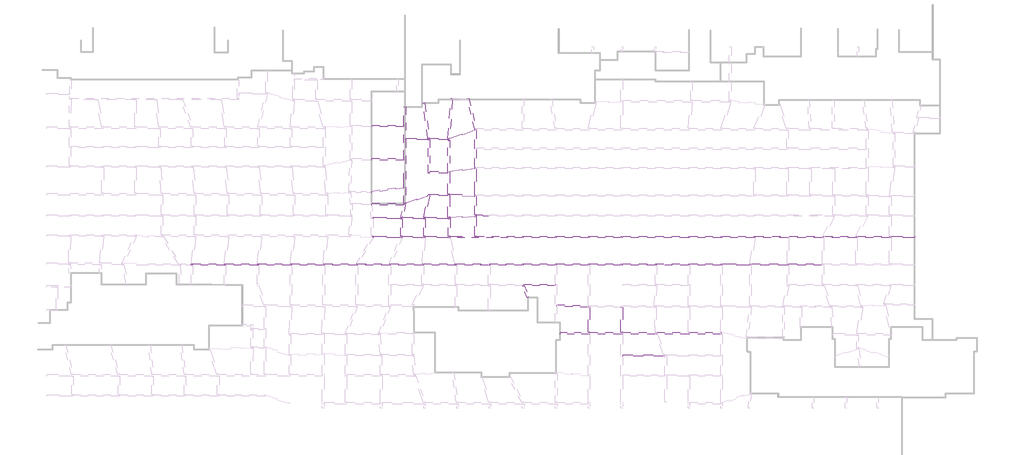
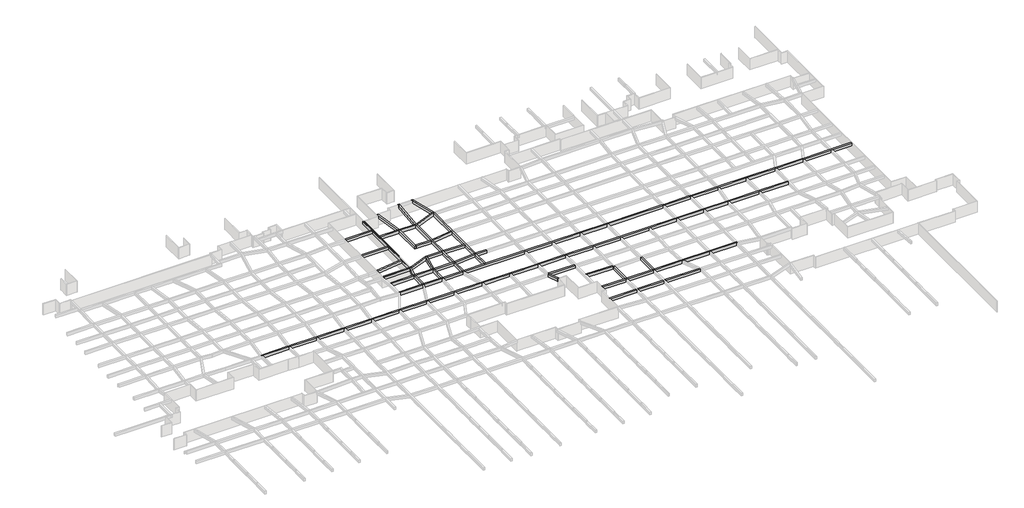
# One storey, part 38 of 45: 38 beams.
"""IFC4 building model written with IfcOpenShell, lengths in millimetres."""

from ifc_helpers import new_model, si_unit, frame, origin, place, context, project, spatial, polyline, outline, extrude, faceted_brep, element, save

model = new_model("IFC4")

# Units and contexts
model_context = context("Model", 3, world=origin())
ifc_project = project(units=[si_unit("LENGTHUNIT", "METRE", prefix="MILLI")], contexts=[model_context])

# Site, building, storey
site = spatial("IfcSite", under=ifc_project)
building = spatial("IfcBuilding", under=site)
storey = spatial("IfcBuildingStorey", under=building, Name="户型图", Elevation=0.0)

# Beams
placement = place(None, origin())
element("IfcBeam", 1, ObjectType="混凝土 - 矩形梁 : KL_beam", at=placement, inside=storey, context=model_context, shape_type="Brep", body=[
    faceted_brep([(-107399.1449794, 152479.7935386, 3300.0), (-107399.1449794, 152079.7935386, 3300.0), (-107019.2456688, 152079.7935386, 3300.0), (-99643.5692432, 152079.7935386, 3300.0), (-99243.5692432, 152079.7935386, 3300.0), (-91843.5387872, 152079.7935386, 3300.0), (-91443.5387872, 152079.7935386, 3300.0), (-84024.3638582, 152079.7935386, 3300.0), (-83624.3638582, 152079.7935386, 3300.0), (-76287.7540188, 152079.7935386, 3300.0), (-75887.7540188, 152079.7935386, 3300.0), (-68487.7540188, 152079.7935386, 3300.0), (-68087.7540188, 152079.7935386, 3300.0), (-60687.7540188, 152079.7935386, 3300.0), (-60287.7540188, 152079.7935386, 3300.0), (-52887.7424309, 152079.7935386, 3300.0), (-52487.7424309, 152079.7935386, 3300.0), (-45087.7540188, 152079.7935386, 3300.0), (-44687.7540188, 152079.7935386, 3300.0), (-37220.6748317, 152079.7935386, 3300.0), (-36820.6748317, 152079.7935386, 3300.0), (-29220.6748317, 152079.7935386, 3300.0), (-28820.6748317, 152079.7935386, 3300.0), (-21420.6748317, 152079.7935386, 3300.0), (-21020.6748317, 152079.7935386, 3300.0), (-13620.6748317, 152079.7935386, 3300.0), (-13220.6748317, 152079.7935386, 3300.0), (-5904.3123934, 152079.7935386, 3300.0), (-5504.3123934, 152079.7935386, 3300.0), (2173.6750398, 152079.7935386, 3300.0), (2573.6750398, 152079.7935386, 3300.0), (9973.3027926, 152079.7935386, 3300.0), (10373.3027926, 152079.7935386, 3300.0), (17658.170888, 152079.7935386, 3300.0), (18058.170888, 152079.7935386, 3300.0), (24544.7928364, 152079.7935386, 3300.0), (24944.7928364, 152079.7935386, 3300.0), (33358.170888, 152079.7935386, 3300.0), (33758.170888, 152079.7935386, 3300.0), (41658.170888, 152079.7935386, 3300.0), (41658.170888, 152479.7935386, 3300.0), (33758.170888, 152479.7935386, 3300.0), (33358.170888, 152479.7935386, 3300.0), (24974.8665178, 152479.7935386, 3300.0), (24570.9354888, 152479.7935386, 3300.0), (18058.170888, 152479.7935386, 3300.0), (17658.170888, 152479.7935386, 3300.0), (10373.3027926, 152479.7935386, 3300.0), (9973.3027926, 152479.7935386, 3300.0), (-5504.3123934, 152479.7935386, 3300.0), (-5904.3123934, 152479.7935386, 3300.0), (-13220.6748317, 152479.7935386, 3300.0), (-13620.6748317, 152479.7935386, 3300.0), (-21020.6748317, 152479.7935386, 3300.0), (-21420.6748317, 152479.7935386, 3300.0), (-28820.6748317, 152479.7935386, 3300.0), (-29220.6748317, 152479.7935386, 3300.0), (-44731.4968935, 152479.7935386, 3300.0), (-45143.7423452, 152479.7935386, 3300.0), (-52476.9979937, 152479.7935386, 3300.0), (-52877.5469321, 152479.7935386, 3300.0), (-60185.5869801, 152479.7935386, 3300.0), (-60620.131131, 152479.7935386, 3300.0), (-67941.3438573, 152479.7935386, 3300.0), (-68403.2240726, 152479.7935386, 3300.0), (-75865.4450548, 152479.7935386, 3300.0), (-76267.6837854, 152479.7935386, 3300.0), (-83602.0244383, 152479.7935386, 3300.0), (-84004.2631688, 152479.7935386, 3300.0), (-91421.2298232, 152479.7935386, 3300.0), (-91823.4685538, 152479.7935386, 3300.0), (-99221.2298232, 152479.7935386, 3300.0), (-99623.4685538, 152479.7935386, 3300.0), (-106996.9062488, 152479.7935386, 3300.0), (-107399.1449794, 152079.7935386, 2500.0), (-107019.2456688, 152079.7935386, 2500.0), (-99643.5692432, 152079.7935386, 2500.0), (-99243.5692432, 152079.7935386, 2500.0), (-91843.5387872, 152079.7935386, 2500.0), (-91443.5387872, 152079.7935386, 2500.0), (-84024.3638582, 152079.7935386, 2500.0), (-83624.3638582, 152079.7935386, 2500.0), (-76287.7540188, 152079.7935386, 2500.0), (-75887.7540188, 152079.7935386, 2500.0), (-68487.7540188, 152079.7935386, 2500.0), (-68087.7540188, 152079.7935386, 2500.0), (-60687.7540188, 152079.7935386, 2500.0), (-60287.7540188, 152079.7935386, 2500.0), (-52887.7424309, 152079.7935386, 2500.0), (-52487.7424309, 152079.7935386, 2500.0), (-45087.7540188, 152079.7935386, 2500.0), (-44687.7540188, 152079.7935386, 2500.0), (-37220.6748317, 152079.7935386, 2500.0), (-36820.6748317, 152079.7935386, 2500.0), (-29220.6748317, 152079.7935386, 2500.0), (-28820.6748317, 152079.7935386, 2500.0), (-21420.6748317, 152079.7935386, 2500.0), (-21020.6748317, 152079.7935386, 2500.0), (-13620.6748317, 152079.7935386, 2500.0), (-13220.6748317, 152079.7935386, 2500.0), (-5904.3123934, 152079.7935386, 2500.0), (-5504.3123934, 152079.7935386, 2500.0), (2173.6750398, 152079.7935386, 2500.0), (2573.6750398, 152079.7935386, 2500.0), (9973.3027926, 152079.7935386, 2500.0), (10373.3027926, 152079.7935386, 2500.0), (17658.170888, 152079.7935386, 2500.0), (18058.170888, 152079.7935386, 2500.0), (24544.7928364, 152079.7935386, 2500.0), (24944.7928364, 152079.7935386, 2500.0), (33358.170888, 152079.7935386, 2500.0), (33758.170888, 152079.7935386, 2500.0), (41658.170888, 152079.7935386, 2500.0), (-107399.1449794, 152479.7935386, 2500.0), (-106996.9062488, 152479.7935386, 2500.0), (-99623.4685538, 152479.7935386, 2500.0), (-99221.2298232, 152479.7935386, 2500.0), (-91823.4685538, 152479.7935386, 2500.0), (-91421.2298232, 152479.7935386, 2500.0), (-84004.2631688, 152479.7935386, 2500.0), (-83602.0244383, 152479.7935386, 2500.0), (-76267.6837854, 152479.7935386, 2500.0), (-75865.4450548, 152479.7935386, 2500.0), (-68403.2240726, 152479.7935386, 2500.0), (-67941.3438573, 152479.7935386, 2500.0), (-60620.131131, 152479.7935386, 2500.0), (-60185.5869801, 152479.7935386, 2500.0), (-52877.5469321, 152479.7935386, 2500.0), (-52476.9979937, 152479.7935386, 2500.0), (-45143.7423452, 152479.7935386, 2500.0), (-44731.4968935, 152479.7935386, 2500.0), (-29220.6748317, 152479.7935386, 2500.0), (-28820.6748317, 152479.7935386, 2500.0), (-21420.6748317, 152479.7935386, 2500.0), (-21020.6748317, 152479.7935386, 2500.0), (-13620.6748317, 152479.7935386, 2500.0), (-13220.6748317, 152479.7935386, 2500.0), (-5904.3123934, 152479.7935386, 2500.0), (-5504.3123934, 152479.7935386, 2500.0), (9973.3027926, 152479.7935386, 2500.0), (10373.3027926, 152479.7935386, 2500.0), (17658.170888, 152479.7935386, 2500.0), (18058.170888, 152479.7935386, 2500.0), (24570.9354888, 152479.7935386, 2500.0), (24974.8665178, 152479.7935386, 2500.0), (33358.170888, 152479.7935386, 2500.0), (33758.170888, 152479.7935386, 2500.0), (41658.170888, 152479.7935386, 2500.0)], [[[0, 1, 2, 3, 4, 5, 6, 7, 8, 9, 10, 11, 12, 13, 14, 15, 16, 17, 18, 19, 20, 21, 22, 23, 24, 25, 26, 27, 28, 29, 30, 31, 32, 33, 34, 35, 36, 37, 38, 39, 40, 41, 42, 43, 44, 45, 46, 47, 48, 49, 50, 51, 52, 53, 54, 55, 56, 57, 58, 59, 60, 61, 62, 63, 64, 65, 66, 67, 68, 69, 70, 71, 72, 73]], [[1, 74, 75, 76, 77, 78, 79, 80, 81, 82, 83, 84, 85, 86, 87, 88, 89, 90, 91, 92, 93, 94, 95, 96, 97, 98, 99, 100, 101, 102, 103, 104, 105, 106, 107, 108, 109, 110, 111, 112, 39, 38, 37, 36, 35, 34, 33, 32, 31, 30, 29, 28, 27, 26, 25, 24, 23, 22, 21, 20, 19, 18, 17, 16, 15, 14, 13, 12, 11, 10, 9, 8, 7, 6, 5, 4, 3, 2]], [[74, 113, 114, 115, 116, 117, 118, 119, 120, 121, 122, 123, 124, 125, 126, 127, 128, 129, 130, 131, 132, 133, 134, 135, 136, 137, 138, 139, 140, 141, 142, 143, 144, 145, 146, 147, 112, 111, 110, 109, 108, 107, 106, 105, 104, 103, 102, 101, 100, 99, 98, 97, 96, 95, 94, 93, 92, 91, 90, 89, 88, 87, 86, 85, 84, 83, 82, 81, 80, 79, 78, 77, 76, 75]], [[113, 0, 73, 72, 71, 70, 69, 68, 67, 66, 65, 64, 63, 62, 61, 60, 59, 58, 57, 56, 55, 54, 53, 52, 51, 50, 49, 48, 47, 46, 45, 44, 43, 42, 41, 40, 147, 146, 145, 144, 143, 142, 141, 140, 139, 138, 137, 136, 135, 134, 133, 132, 131, 130, 129, 128, 127, 126, 125, 124, 123, 122, 121, 120, 119, 118, 117, 116, 115, 114]], [[0, 113, 74, 1]], [[40, 39, 112, 147]]]),
])
element("IfcBeam", 2, ObjectType="混凝土 - 矩形梁 : KL_beam", at=placement, inside=storey, context=model_context, shape_type="Brep", body=[
    faceted_brep([(63459.1822514, 158978.3181414, 3300.0), (63459.1822514, 158578.3181414, 3300.0), (63459.1822514, 158578.3181414, 2500.0), (63459.1822514, 158978.3181414, 2500.0), (57931.1254195, 158978.3181414, 3300.0), (57531.1254195, 158978.3181414, 3300.0), (50062.8813826, 158978.3181414, 3300.0), (49613.9508875, 158978.3181414, 3300.0), (42278.2377938, 158978.3181414, 3300.0), (41833.1970176, 158978.3181414, 3300.0), (25858.170888, 158978.3181414, 3300.0), (25458.170888, 158978.3181414, 3300.0), (18058.170888, 158978.3181414, 3300.0), (17658.170888, 158978.3181414, 3300.0), (10373.3027926, 158978.3181414, 3300.0), (9973.3027926, 158978.3181414, 3300.0), (-5504.3123934, 158978.3181414, 3300.0), (-5904.3123934, 158978.3181414, 3300.0), (-13220.6748317, 158978.3181414, 3300.0), (-13620.6748317, 158978.3181414, 3300.0), (-21020.6748317, 158978.3181414, 3300.0), (-21420.6748317, 158978.3181414, 3300.0), (-28820.6748317, 158978.3181414, 3300.0), (-29220.6748317, 158978.3181414, 3300.0), (-40021.1080966, 158978.3181414, 3300.0), (-40421.1080966, 158978.3181414, 3300.0), (-46244.2344007, 158978.3181414, 3300.0), (-46644.2344007, 158978.3181414, 3300.0), (-52129.2939824, 158978.3181414, 3300.0), (-52529.2939824, 158978.3181414, 3300.0), (-57529.2939824, 158978.3181414, 3300.0), (-57929.2939824, 158978.3181414, 3300.0), (-64444.2344007, 158978.3181414, 3300.0), (-64637.1523876, 158978.3181414, 3300.0), (-64301.3522933, 158784.4438666, 3300.0), (-64420.3590362, 158578.3181414, 3300.0), (-58031.4610211, 158578.3181414, 3300.0), (-57596.9168701, 158578.3181414, 3300.0), (-52557.9368008, 158578.3181414, 3300.0), (-52157.3878624, 158578.3181414, 3300.0), (-46664.2753047, 158578.3181414, 3300.0), (-46252.029853, 158578.3181414, 3300.0), (-46244.2344007, 158578.3181414, 3300.0), (-29220.6748317, 158578.3181414, 3300.0), (-28820.6748317, 158578.3181414, 3300.0), (-21420.6748317, 158578.3181414, 3300.0), (-21020.6748317, 158578.3181414, 3300.0), (-13620.6748317, 158578.3181414, 3300.0), (-13220.6748317, 158578.3181414, 3300.0), (-5904.3123934, 158578.3181414, 3300.0), (-5504.3123934, 158578.3181414, 3300.0), (9973.3027926, 158578.3181414, 3300.0), (10373.3027926, 158578.3181414, 3300.0), (17658.170888, 158578.3181414, 3300.0), (18058.170888, 158578.3181414, 3300.0), (25428.027227, 158578.3181414, 3300.0), (25831.958256, 158578.3181414, 3300.0), (33358.170888, 158578.3181414, 3300.0), (33758.170888, 158578.3181414, 3300.0), (41658.170888, 158578.3181414, 3300.0), (42058.170888, 158578.3181414, 3300.0), (49536.7318858, 158578.3181414, 3300.0), (49936.7318858, 158578.3181414, 3300.0), (57531.1254195, 158578.3181414, 3300.0), (57931.1254195, 158578.3181414, 3300.0), (-64420.3590362, 158578.3181414, 2500.0), (-58031.4610211, 158578.3181414, 2500.0), (-57596.9168701, 158578.3181414, 2500.0), (-52557.9368008, 158578.3181414, 2500.0), (-52157.3878624, 158578.3181414, 2500.0), (-46664.2753047, 158578.3181414, 2500.0), (-46252.029853, 158578.3181414, 2500.0), (-46244.2344007, 158578.3181414, 2500.0), (-29220.6748317, 158578.3181414, 2500.0), (-28820.6748317, 158578.3181414, 2500.0), (-21420.6748317, 158578.3181414, 2500.0), (-21020.6748317, 158578.3181414, 2500.0), (-13620.6748317, 158578.3181414, 2500.0), (-13220.6748317, 158578.3181414, 2500.0), (-5904.3123934, 158578.3181414, 2500.0), (-5504.3123934, 158578.3181414, 2500.0), (9973.3027926, 158578.3181414, 2500.0), (10373.3027926, 158578.3181414, 2500.0), (17658.170888, 158578.3181414, 2500.0), (18058.170888, 158578.3181414, 2500.0), (25428.027227, 158578.3181414, 2500.0), (25831.958256, 158578.3181414, 2500.0), (33358.170888, 158578.3181414, 2500.0), (33758.170888, 158578.3181414, 2500.0), (41658.170888, 158578.3181414, 2500.0), (42058.170888, 158578.3181414, 2500.0), (49536.7318858, 158578.3181414, 2500.0), (49936.7318858, 158578.3181414, 2500.0), (57531.1254195, 158578.3181414, 2500.0), (57931.1254195, 158578.3181414, 2500.0), (-64301.3522933, 158784.4438666, 2500.0), (-64637.1523876, 158978.3181414, 2500.0), (-64444.2344007, 158978.3181414, 2500.0), (-57929.2939824, 158978.3181414, 2500.0), (-57529.2939824, 158978.3181414, 2500.0), (-52529.2939824, 158978.3181414, 2500.0), (-52129.2939824, 158978.3181414, 2500.0), (-46644.2344007, 158978.3181414, 2500.0), (-46244.2344007, 158978.3181414, 2500.0), (-40421.1080966, 158978.3181414, 2500.0), (-40021.1080966, 158978.3181414, 2500.0), (-29220.6748317, 158978.3181414, 2500.0), (-28820.6748317, 158978.3181414, 2500.0), (-21420.6748317, 158978.3181414, 2500.0), (-21020.6748317, 158978.3181414, 2500.0), (-13620.6748317, 158978.3181414, 2500.0), (-13220.6748317, 158978.3181414, 2500.0), (-5904.3123934, 158978.3181414, 2500.0), (-5504.3123934, 158978.3181414, 2500.0), (9973.3027926, 158978.3181414, 2500.0), (10373.3027926, 158978.3181414, 2500.0), (17658.170888, 158978.3181414, 2500.0), (18058.170888, 158978.3181414, 2500.0), (25458.170888, 158978.3181414, 2500.0), (25858.170888, 158978.3181414, 2500.0), (41833.1970176, 158978.3181414, 2500.0), (42278.2377938, 158978.3181414, 2500.0), (49613.9508875, 158978.3181414, 2500.0), (50062.8813826, 158978.3181414, 2500.0), (57531.1254195, 158978.3181414, 2500.0), (57931.1254195, 158978.3181414, 2500.0)], [[[0, 1, 2, 3]], [[1, 0, 4, 5, 6, 7, 8, 9, 10, 11, 12, 13, 14, 15, 16, 17, 18, 19, 20, 21, 22, 23, 24, 25, 26, 27, 28, 29, 30, 31, 32, 33, 34, 35, 36, 37, 38, 39, 40, 41, 42, 43, 44, 45, 46, 47, 48, 49, 50, 51, 52, 53, 54, 55, 56, 57, 58, 59, 60, 61, 62, 63, 64]], [[2, 1, 64, 63, 62, 61, 60, 59, 58, 57, 56, 55, 54, 53, 52, 51, 50, 49, 48, 47, 46, 45, 44, 43, 42, 41, 40, 39, 38, 37, 36, 35, 65, 66, 67, 68, 69, 70, 71, 72, 73, 74, 75, 76, 77, 78, 79, 80, 81, 82, 83, 84, 85, 86, 87, 88, 89, 90, 91, 92, 93, 94]], [[3, 2, 94, 93, 92, 91, 90, 89, 88, 87, 86, 85, 84, 83, 82, 81, 80, 79, 78, 77, 76, 75, 74, 73, 72, 71, 70, 69, 68, 67, 66, 65, 95, 96, 97, 98, 99, 100, 101, 102, 103, 104, 105, 106, 107, 108, 109, 110, 111, 112, 113, 114, 115, 116, 117, 118, 119, 120, 121, 122, 123, 124, 125]], [[0, 3, 125, 124, 123, 122, 121, 120, 119, 118, 117, 116, 115, 114, 113, 112, 111, 110, 109, 108, 107, 106, 105, 104, 103, 102, 101, 100, 99, 98, 97, 96, 33, 32, 31, 30, 29, 28, 27, 26, 25, 24, 23, 22, 21, 20, 19, 18, 17, 16, 15, 14, 13, 12, 11, 10, 9, 8, 7, 6, 5, 4]], [[34, 95, 65, 35]], [[95, 34, 33, 96]]]),
])
element("IfcBeam", 3, ObjectType="混凝土 - 矩形梁 : KL_beam", at=placement, inside=storey, context=model_context, shape_type="Brep", body=[
    faceted_brep([(-64444.2344007, 163210.8437885, 3300.0), (-64444.2344007, 163000.3622326, 3300.0), (-57929.2939824, 163000.3622326, 3300.0), (-57529.2939824, 163000.3622326, 3300.0), (-52529.2939824, 163000.3622326, 3300.0), (-52129.2939824, 163000.3622326, 3300.0), (-46644.2344007, 163000.3622326, 3300.0), (-46244.2344007, 163000.3622326, 3300.0), (-46244.2344007, 163018.5507812, 3300.0), (-46244.2344007, 163400.3622326, 3300.0), (-46344.2344007, 163400.3622326, 3300.0), (-46744.2344007, 163400.3622326, 3300.0), (-52086.6745815, 163400.3622326, 3300.0), (-52494.1612595, 163400.3622326, 3300.0), (-57477.854433, 163400.3622326, 3300.0), (-57888.3760761, 163400.3622326, 3300.0), (-64464.1535918, 163400.3622326, 3300.0), (-64444.2344007, 163000.3622326, 2500.0), (-57929.2939824, 163000.3622326, 2500.0), (-57529.2939824, 163000.3622326, 2500.0), (-52529.2939824, 163000.3622326, 2500.0), (-52129.2939824, 163000.3622326, 2500.0), (-46644.2344007, 163000.3622326, 2500.0), (-46244.2344007, 163000.3622326, 2500.0), (-64444.2344007, 163210.8437885, 2500.0), (-64464.1535918, 163400.3622326, 2500.0), (-57888.3760761, 163400.3622326, 2500.0), (-57477.854433, 163400.3622326, 2500.0), (-52494.1612595, 163400.3622326, 2500.0), (-52086.6745815, 163400.3622326, 2500.0), (-46744.2344007, 163400.3622326, 2500.0), (-46344.2344007, 163400.3622326, 2500.0), (-46244.2344007, 163400.3622326, 2500.0), (-46244.2344007, 163018.5507812, 2500.0)], [[[0, 1, 2, 3, 4, 5, 6, 7, 8, 9, 10, 11, 12, 13, 14, 15, 16]], [[1, 17, 18, 19, 20, 21, 22, 23, 7, 6, 5, 4, 3, 2]], [[17, 24, 25, 26, 27, 28, 29, 30, 31, 32, 33, 23, 22, 21, 20, 19, 18]], [[9, 32, 31, 30, 29, 28, 27, 26, 25, 16, 15, 14, 13, 12, 11, 10]], [[1, 0, 24, 17]], [[0, 16, 25, 24]], [[9, 8, 7, 23, 33, 32]]]),
])
element("IfcBeam", 4, ObjectType="混凝土 - 矩形梁 : KL_beam", at=placement, inside=storey, context=model_context, shape_type="SweptSolid", body=[
    extrude(outline(polyline([(-57529.2939824, 158978.3181414), (-57929.2939824, 158978.3181414), (-57929.2939824, 163000.3622326), (-57529.2939824, 163000.3622326), (-57529.2939824, 158978.3181414)])), frame((0.0, 0.0, 2500.0), z_axis=(0.0, 0.0, 1.0), x_axis=(1.0, 0.0, 0.0)), (0.0, 0.0, 1.0), 800.0),
])
element("IfcBeam", 5, ObjectType="混凝土 - 矩形梁 : KL_beam", at=placement, inside=storey, context=model_context, shape_type="SweptSolid", body=[
    extrude(outline(polyline([(-52129.2939824, 158978.3181414), (-52529.2939824, 158978.3181414), (-52529.2939824, 163000.3622326), (-52129.2939824, 163000.3622326), (-52129.2939824, 158978.3181414)])), frame((0.0, 0.0, 2500.0), z_axis=(0.0, 0.0, 1.0), x_axis=(1.0, 0.0, 0.0)), (0.0, 0.0, 1.0), 800.0),
])
element("IfcBeam", 6, ObjectType="混凝土 - 矩形梁 : KL_beam", at=placement, inside=storey, context=model_context, shape_type="SweptSolid", body=[
    extrude(outline(polyline([(-46644.2344007, 163000.3622326), (-46244.2344007, 163000.3622326), (-46244.2344007, 158978.3181414), (-46644.2344007, 158978.3181414), (-46644.2344007, 163000.3622326)])), frame((0.0, 0.0, 2500.0), z_axis=(0.0, 0.0, 1.0), x_axis=(1.0, 0.0, 0.0)), (0.0, 0.0, 1.0), 800.0),
    extrude(outline(polyline([(-46244.2344007, 158547.0522899), (-46252.029853, 158578.3181414), (-46244.2344007, 158578.3181414), (-46244.2344007, 158547.0522899)])), frame((0.0, 0.0, 2500.0), z_axis=(0.0, 0.0, 1.0), x_axis=(1.0, 0.0, 0.0)), (0.0, 0.0, 1.0), 800.0),
])
element("IfcBeam", 7, ObjectType="混凝土 - 矩形梁 : KL_beam", at=placement, inside=storey, context=model_context, shape_type="Brep", body=[
    faceted_brep([(-56685.1558367, 166833.9170778, 3300.0), (-56771.3878839, 166800.8872671, 3300.0), (-57081.0281845, 166682.2844873, 3300.0), (-57135.5017388, 166661.419261, 3300.0), (-57223.0318982, 166282.2844873, 3300.0), (-57888.3760761, 163400.3622326, 3300.0), (-57477.854433, 163400.3622326, 3300.0), (-56793.6389178, 166364.0252292, 3300.0), (-56685.1558367, 166833.9170778, 2500.0), (-57477.854433, 163400.3622326, 2500.0), (-56793.6389178, 166364.0252292, 2500.0), (-57135.5017388, 166661.419261, 2500.0), (-57081.0281845, 166682.2844873, 2500.0), (-56771.3878839, 166800.8872671, 2500.0), (-57888.3760761, 163400.3622326, 2500.0), (-57223.0318982, 166282.2844873, 2500.0)], [[[0, 1, 2, 3, 4, 5, 6, 7]], [[8, 0, 7, 6, 9, 10]], [[11, 12, 13, 8, 10, 9, 14, 15]], [[3, 11, 15, 14, 5, 4]], [[6, 5, 14, 9]], [[3, 2, 1, 0, 8, 13, 12, 11]]]),
])
element("IfcBeam", 8, ObjectType="混凝土 - 矩形梁 : KL_beam", at=placement, inside=storey, context=model_context, shape_type="Brep", body=[
    faceted_brep([(-51297.7565778, 168897.4744599, 3300.0), (-51435.9175617, 168844.5540981, 3300.0), (-51525.8760493, 168381.7577996, 3300.0), (-52494.1612595, 163400.3622326, 3300.0), (-52086.6745815, 163400.3622326, 3300.0), (-51095.8963311, 168497.4744599, 3300.0), (-51018.1442074, 168897.4744599, 3300.0), (-51018.1442074, 168897.4744599, 2500.0), (-52086.6745815, 163400.3622326, 2500.0), (-51095.8963311, 168497.4744599, 2500.0), (-51435.9175617, 168844.5540981, 2500.0), (-51297.7565778, 168897.4744599, 2500.0), (-52494.1612595, 163400.3622326, 2500.0), (-51525.8760493, 168381.7577996, 2500.0)], [[[0, 1, 2, 3, 4, 5, 6]], [[7, 6, 5, 4, 8, 9]], [[10, 11, 7, 9, 8, 12, 13]], [[1, 10, 13, 12, 3, 2]], [[4, 3, 12, 8]], [[0, 11, 10, 1]], [[11, 0, 6, 7]]]),
])
element("IfcBeam", 9, ObjectType="混凝土 - 矩形梁 : KL_beam", at=placement, inside=storey, context=model_context, shape_type="Brep", body=[
    faceted_brep([(-46344.2344007, 168897.4744599, 3300.0), (-46344.4990045, 168897.4744599, 3300.0), (-46541.0079915, 168897.4744599, 3300.0), (-46744.2344007, 168897.4744599, 3300.0), (-46744.2344007, 168497.4744599, 3300.0), (-46744.2344007, 163400.3622326, 3300.0), (-46344.2344007, 163400.3622326, 3300.0), (-46344.2344007, 163410.8212036, 3300.0), (-46344.2344007, 168490.359157, 3300.0), (-46344.2344007, 168890.6029747, 3300.0), (-46344.2344007, 168897.4744599, 2500.0), (-46344.2344007, 163400.3622326, 2500.0), (-46344.2344007, 163410.8212036, 2500.0), (-46344.2344007, 168490.359157, 2500.0), (-46344.2344007, 168890.6029747, 2500.0), (-46744.2344007, 168897.4744599, 2500.0), (-46541.0079915, 168897.4744599, 2500.0), (-46344.4990045, 168897.4744599, 2500.0), (-46744.2344007, 163400.3622326, 2500.0), (-46744.2344007, 168497.4744599, 2500.0)], [[[0, 1, 2, 3, 4, 5, 6, 7, 8, 9]], [[10, 0, 9, 8, 7, 6, 11, 12, 13, 14]], [[15, 16, 17, 10, 14, 13, 12, 11, 18, 19]], [[3, 15, 19, 18, 5, 4]], [[6, 5, 18, 11]], [[3, 2, 1, 0, 10, 17, 16, 15]]]),
])
element("IfcBeam", 10, ObjectType="混凝土 - 矩形梁 : KL_beam", at=placement, inside=storey, context=model_context, shape_type="SweptSolid", body=[
    extrude(outline(polyline([(-56793.6389178, 166364.0252292), (-56685.1558367, 166833.9170778), (-51435.9175617, 168844.5540981), (-51525.8760493, 168381.7577996), (-56793.6389178, 166364.0252292)])), frame((0.0, 0.0, 2500.0), z_axis=(0.0, 0.0, 1.0), x_axis=(1.0, 0.0, 0.0)), (0.0, 0.0, 1.0), 800.0),
])
element("IfcBeam", 11, ObjectType="混凝土 - 矩形梁 : KL_beam", at=placement, inside=storey, context=model_context, shape_type="Brep", body=[
    faceted_brep([(-51018.1442074, 168897.4744599, 3300.0), (-51085.6096548, 168550.3948218, 3300.0), (-51095.8963311, 168497.4744599, 3300.0), (-46744.2344007, 168497.4744599, 3300.0), (-46744.2344007, 168897.4744599, 3300.0), (-46744.4990045, 168897.4744599, 3300.0), (-51095.8963311, 168497.4744599, 2500.0), (-46744.2344007, 168497.4744599, 2500.0), (-51085.6096548, 168550.3948218, 2500.0), (-51018.1442074, 168897.4744599, 2500.0), (-46744.4990045, 168897.4744599, 2500.0), (-46744.2344007, 168897.4744599, 2500.0)], [[[0, 1, 2, 3, 4, 5]], [[2, 6, 7, 3]], [[6, 8, 9, 10, 11, 7]], [[9, 0, 5, 4, 11, 10]], [[6, 2, 1, 0, 9, 8]], [[4, 3, 7, 11]]]),
])
element("IfcBeam", 12, ObjectType="混凝土 - 矩形梁 : KL_beam", at=placement, inside=storey, context=model_context, shape_type="Brep", body=[
    faceted_brep([(-46344.2344007, 168890.6029747, 3300.0), (-46344.2344007, 168490.359157, 3300.0), (-40420.6748317, 168283.5038987, 3300.0), (-40420.6748317, 168683.7477164, 3300.0), (-46344.2344007, 168490.359157, 2500.0), (-40420.6748317, 168283.5038987, 2500.0), (-46344.2344007, 168890.6029747, 2500.0), (-40420.6748317, 168683.7477164, 2500.0)], [[[0, 1, 2, 3]], [[1, 4, 5, 2]], [[4, 6, 7, 5]], [[6, 0, 3, 7]], [[0, 6, 4, 1]], [[3, 2, 5, 7]]]),
    faceted_brep([(-46541.0079915, 168897.4744599, 2500.0), (-46541.0079915, 168897.4744599, 3300.0), (-46744.2344007, 168897.4744599, 3300.0), (-46744.4990045, 168897.4744599, 3300.0), (-46744.4990045, 168897.4744599, 2500.0), (-46744.2344007, 168897.4744599, 2500.0), (-46744.4990045, 168904.5805227, 3300.0), (-46744.4990045, 168904.5805227, 2500.0)], [[[0, 1, 2, 3, 4, 5]], [[6, 7, 4, 3]], [[1, 6, 3, 2]], [[7, 0, 5, 4]], [[1, 0, 7, 6]]]),
])
element("IfcBeam", 13, ObjectType="混凝土 - 矩形梁 : KL_beam", at=placement, inside=storey, context=model_context, shape_type="Brep", body=[
    faceted_brep([(-46244.2344007, 163400.3622326, 3300.0), (-46244.2344007, 163018.5507812, 3300.0), (-40421.1080966, 163574.6111972, 3300.0), (-40021.1080966, 163612.8078899, 3300.0), (-40020.6748317, 163612.8492632, 3300.0), (-40020.6748317, 163994.4687414, 3300.0), (-40020.6748317, 164014.6688587, 3300.0), (-40420.6748317, 163976.4721659, 3300.0), (-46344.2344007, 163410.8212036, 3300.0), (-46344.2344007, 163400.3622326, 3300.0), (-46244.2344007, 163018.5507812, 2500.0), (-40421.1080966, 163574.6111972, 2500.0), (-40021.1080966, 163612.8078899, 2500.0), (-40020.6748317, 163612.8492632, 2500.0), (-46244.2344007, 163400.3622326, 2500.0), (-46344.2344007, 163400.3622326, 2500.0), (-46344.2344007, 163410.8212036, 2500.0), (-40420.6748317, 163976.4721659, 2500.0), (-40020.6748317, 164014.6688587, 2500.0), (-40020.6748317, 163994.4687414, 2500.0)], [[[0, 1, 2, 3, 4, 5, 6, 7, 8, 9]], [[1, 10, 11, 12, 13, 4, 3, 2]], [[10, 14, 15, 16, 17, 18, 19, 13, 12, 11]], [[6, 18, 17, 16, 8, 7]], [[0, 14, 10, 1]], [[14, 0, 9, 15]], [[9, 8, 16, 15]], [[6, 5, 4, 13, 19, 18]]]),
])
element("IfcBeam", 14, ObjectType="混凝土 - 矩形梁 : KL_beam", at=placement, inside=storey, context=model_context, shape_type="Brep", body=[
    faceted_brep([(-40020.6748317, 184219.2176267, 3300.0), (-40420.6748317, 184170.1038023, 3300.0), (-40420.6748317, 183903.6589088, 3300.0), (-40420.6748317, 175230.1542355, 3300.0), (-40420.6748317, 174825.1839588, 3300.0), (-40420.6748317, 168683.7477164, 3300.0), (-40420.6748317, 168283.5038987, 3300.0), (-40420.6748317, 163976.4721659, 3300.0), (-40020.6748317, 164014.6688587, 3300.0), (-40020.6748317, 168316.2365071, 3300.0), (-40020.6748317, 168716.2365071, 3300.0), (-40020.6748317, 174859.2955299, 3300.0), (-40020.6748317, 175259.2955299, 3300.0), (-40020.6748317, 179411.4368869, 3300.0), (-40020.6748317, 179811.4368869, 3300.0), (-40020.6748317, 183994.3140025, 3300.0), (-40020.6748317, 184219.2176267, 2500.0), (-40020.6748317, 164014.6688587, 2500.0), (-40020.6748317, 168316.2365071, 2500.0), (-40020.6748317, 168716.2365071, 2500.0), (-40020.6748317, 174859.2955299, 2500.0), (-40020.6748317, 175259.2955299, 2500.0), (-40020.6748317, 179411.4368869, 2500.0), (-40020.6748317, 179811.4368869, 2500.0), (-40020.6748317, 183994.3140025, 2500.0), (-40420.6748317, 184170.1038023, 2500.0), (-40420.6748317, 163976.4721659, 2500.0), (-40420.6748317, 168283.5038987, 2500.0), (-40420.6748317, 168683.7477164, 2500.0), (-40420.6748317, 174825.1839588, 2500.0), (-40420.6748317, 175230.1542355, 2500.0), (-40420.6748317, 183903.6589088, 2500.0)], [[[0, 1, 2, 3, 4, 5, 6, 7, 8, 9, 10, 11, 12, 13, 14, 15]], [[16, 0, 15, 14, 13, 12, 11, 10, 9, 8, 17, 18, 19, 20, 21, 22, 23, 24]], [[25, 16, 24, 23, 22, 21, 20, 19, 18, 17, 26, 27, 28, 29, 30, 31]], [[1, 25, 31, 30, 29, 28, 27, 26, 7, 6, 5, 4, 3, 2]], [[8, 7, 26, 17]], [[1, 0, 16, 25]]]),
])
element("IfcBeam", 15, ObjectType="混凝土 - 矩形梁 : KL_beam", at=placement, inside=storey, context=model_context, shape_type="Brep", body=[
    faceted_brep([(-40420.6748317, 184170.1038023, 3300.0), (-40020.6748317, 184219.2176267, 3300.0), (-40064.3312613, 184394.3140025, 3300.0), (-41844.548046, 191534.3735401, 3300.0), (-42256.7934978, 191534.3735401, 3300.0), (-42157.0622966, 191134.3735401, 3300.0), (-40457.5408595, 184317.965364, 3300.0), (-40020.6748317, 184219.2176267, 2500.0), (-40064.3312613, 184394.3140025, 2500.0), (-41844.548046, 191534.3735401, 2500.0), (-40420.6748317, 184170.1038023, 2500.0), (-40457.5408595, 184317.965364, 2500.0), (-42157.0622966, 191134.3735401, 2500.0), (-42256.7934978, 191534.3735401, 2500.0)], [[[0, 1, 2, 3, 4, 5, 6]], [[1, 7, 8, 9, 3, 2]], [[7, 10, 11, 12, 13, 9, 8]], [[10, 0, 6, 5, 4, 13, 12, 11]], [[0, 10, 7, 1]], [[4, 3, 9, 13]]]),
])
element("IfcBeam", 16, ObjectType="混凝土 - 矩形梁 : KL_beam", at=placement, inside=storey, context=model_context, shape_type="Brep", body=[
    faceted_brep([(-46616.2994071, 181525.3814597, 3300.0), (-46344.4990045, 181629.715859, 3300.0), (-40420.6748317, 183903.6589088, 3300.0), (-40420.6748317, 184170.1038023, 3300.0), (-40457.5408595, 184317.965364, 3300.0), (-46347.6097756, 182056.9797433, 3300.0), (-46759.6465869, 181898.8136303, 3300.0), (-46667.7042024, 181659.2955299, 3300.0), (-46759.6465869, 181898.8136303, 2500.0), (-40457.5408595, 184317.965364, 2500.0), (-46347.6097756, 182056.9797433, 2500.0), (-40420.6748317, 183903.6589088, 2500.0), (-46344.4990045, 181629.715859, 2500.0), (-46616.2994071, 181525.3814597, 2500.0), (-46667.7042024, 181659.2955299, 2500.0), (-40420.6748317, 184170.1038023, 2500.0)], [[[0, 1, 2, 3, 4, 5, 6, 7]], [[8, 6, 5, 4, 9, 10]], [[11, 12, 13, 14, 8, 10, 9, 15]], [[2, 1, 0, 13, 12, 11]], [[3, 2, 11, 15]], [[4, 3, 15, 9]], [[0, 7, 6, 8, 14, 13]]]),
])
element("IfcBeam", 17, ObjectType="混凝土 - 矩形梁 : KL_beam", at=placement, inside=storey, context=model_context, shape_type="Brep", body=[
    faceted_brep([(-45684.8858419, 191534.3735401, 3300.0), (-46085.8626011, 191534.3735401, 3300.0), (-46748.4245993, 182059.2955299, 3300.0), (-46759.6465869, 181898.8136303, 3300.0), (-46347.6097756, 182056.9797433, 3300.0), (-45712.8565667, 191134.3735401, 3300.0), (-45684.8858419, 191534.3735401, 2500.0), (-46347.6097756, 182056.9797433, 2500.0), (-45712.8565667, 191134.3735401, 2500.0), (-46085.8626011, 191534.3735401, 2500.0), (-46759.6465869, 181898.8136303, 2500.0), (-46748.4245993, 182059.2955299, 2500.0)], [[[0, 1, 2, 3, 4, 5]], [[6, 0, 5, 4, 7, 8]], [[9, 6, 8, 7, 10, 11]], [[1, 9, 11, 10, 3, 2]], [[4, 3, 10, 7]], [[1, 0, 6, 9]]]),
])
element("IfcBeam", 18, ObjectType="混凝土 - 矩形梁 : KL_beam", at=placement, inside=storey, context=model_context, shape_type="Brep", body=[
    faceted_brep([(-46759.6465869, 181898.8136303, 3300.0), (-46748.4245993, 182059.2955299, 3300.0), (-51088.0642345, 182059.2955299, 3300.0), (-51461.9215821, 182059.2955299, 3300.0), (-51461.9215821, 181845.3101675, 3300.0), (-51461.9215821, 181659.2955299, 3300.0), (-51061.9215821, 181659.2955299, 3300.0), (-46744.4990045, 181659.2955299, 3300.0), (-46667.7042024, 181659.2955299, 3300.0), (-46748.4245993, 182059.2955299, 2500.0), (-51088.0642345, 182059.2955299, 2500.0), (-51461.9215821, 182059.2955299, 2500.0), (-46759.6465869, 181898.8136303, 2500.0), (-46667.7042024, 181659.2955299, 2500.0), (-46744.4990045, 181659.2955299, 2500.0), (-51061.9215821, 181659.2955299, 2500.0), (-51461.9215821, 181659.2955299, 2500.0), (-51461.9215821, 181845.3101675, 2500.0)], [[[0, 1, 2, 3, 4, 5, 6, 7, 8]], [[1, 9, 10, 11, 3, 2]], [[9, 12, 13, 14, 15, 16, 17, 11, 10]], [[13, 8, 7, 6, 5, 16, 15, 14]], [[0, 12, 9, 1]], [[12, 0, 8, 13]], [[5, 4, 3, 11, 17, 16]]]),
])
element("IfcBeam", 19, ObjectType="混凝土 - 矩形梁 : KL_beam", at=placement, inside=storey, context=model_context, shape_type="Brep", body=[
    faceted_brep([(-51461.9215821, 173859.2955299, 3300.0), (-51061.9215821, 173859.2955299, 3300.0), (-51061.9215821, 174259.2955299, 3300.0), (-51061.9215821, 181659.2955299, 3300.0), (-51461.9215821, 181659.2955299, 3300.0), (-51461.9215821, 173859.2955299, 2500.0), (-51461.9215821, 181659.2955299, 2500.0), (-51061.9215821, 173859.2955299, 2500.0), (-51061.9215821, 181659.2955299, 2500.0), (-51061.9215821, 174259.2955299, 2500.0)], [[[0, 1, 2, 3, 4]], [[5, 0, 4, 6]], [[7, 5, 6, 8, 9]], [[1, 7, 9, 8, 3, 2]], [[4, 3, 8, 6]], [[1, 0, 5, 7]]]),
])
element("IfcBeam", 20, ObjectType="混凝土 - 矩形梁 : KL_beam", at=placement, inside=storey, context=model_context, shape_type="SweptSolid", body=[
    extrude(outline(polyline([(-51061.9215821, 173859.2955299), (-51061.9215821, 174259.2955299), (-46744.4990045, 174259.2955299), (-46744.4990045, 173859.2955299), (-51061.9215821, 173859.2955299)])), frame((0.0, 0.0, 2500.0), z_axis=(0.0, 0.0, 1.0), x_axis=(1.0, 0.0, 0.0)), (0.0, 0.0, 1.0), 800.0),
])
element("IfcBeam", 21, ObjectType="混凝土 - 矩形梁 : KL_beam", at=placement, inside=storey, context=model_context, shape_type="Brep", body=[
    faceted_brep([(-46344.4990045, 168897.4744599, 3300.0), (-46344.4990045, 173888.4368243, 3300.0), (-46344.4990045, 174293.407101, 3300.0), (-46344.4990045, 181629.715859, 3300.0), (-46616.2994071, 181525.3814597, 3300.0), (-46667.7042024, 181659.2955299, 3300.0), (-46744.4990045, 181659.2955299, 3300.0), (-46744.4990045, 174259.2955299, 3300.0), (-46744.4990045, 173859.2955299, 3300.0), (-46744.4990045, 168904.5805227, 3300.0), (-46541.0079915, 168897.4744599, 3300.0), (-46344.4990045, 168897.4744599, 2500.0), (-46344.4990045, 173888.4368243, 2500.0), (-46344.4990045, 174293.407101, 2500.0), (-46344.4990045, 181629.715859, 2500.0), (-46541.0079915, 168897.4744599, 2500.0), (-46744.4990045, 168904.5805227, 2500.0), (-46744.4990045, 173859.2955299, 2500.0), (-46744.4990045, 174259.2955299, 2500.0), (-46744.4990045, 181659.2955299, 2500.0), (-46667.7042024, 181659.2955299, 2500.0), (-46616.2994071, 181525.3814597, 2500.0)], [[[0, 1, 2, 3, 4, 5, 6, 7, 8, 9, 10]], [[0, 11, 12, 13, 14, 3, 2, 1]], [[14, 13, 12, 11, 15, 16, 17, 18, 19, 20, 21]], [[16, 9, 8, 7, 6, 19, 18, 17]], [[11, 0, 10, 15]], [[21, 4, 3, 14]], [[4, 21, 20, 5]], [[10, 9, 16, 15]], [[6, 5, 20, 19]]]),
])
element("IfcBeam", 22, ObjectType="混凝土 - 矩形梁 : KL_beam", at=placement, inside=storey, context=model_context, shape_type="Brep", body=[
    faceted_brep([(-52656.8638641, 190347.7663009, 3300.0), (-52260.7566366, 190403.4355413, 3300.0), (-52260.7566366, 190403.4355413, 2500.0), (-52656.8638641, 190347.7663009, 2500.0), (-51491.9952635, 182059.2955299, 3300.0), (-51461.9215821, 181845.3101675, 3300.0), (-51461.9215821, 182059.2955299, 3300.0), (-51088.0642345, 182059.2955299, 3300.0), (-51088.0642345, 182059.2955299, 2500.0), (-51461.9215821, 182059.2955299, 2500.0), (-51461.9215821, 181845.3101675, 2500.0), (-51491.9952635, 182059.2955299, 2500.0)], [[[0, 1, 2, 3]], [[1, 0, 4, 5, 6, 7]], [[2, 1, 7, 8]], [[3, 2, 8, 9, 10, 11]], [[0, 3, 11, 10, 5, 4]], [[6, 9, 8, 7]], [[9, 6, 5, 10]]]),
])
element("IfcBeam", 23, ObjectType="混凝土 - 矩形梁 : KL_beam", at=placement, inside=storey, context=model_context, shape_type="SweptSolid", body=[
    extrude(outline(polyline([(-51461.9215821, 181845.3101675), (-51461.9215821, 181659.2955299), (-56771.3878839, 181659.2955299), (-56771.3878839, 182059.2955299), (-51491.9952635, 182059.2955299), (-51461.9215821, 181845.3101675)])), frame((0.0, 0.0, 2500.0), z_axis=(0.0, 0.0, 1.0), x_axis=(1.0, 0.0, 0.0)), (0.0, 0.0, 1.0), 800.0),
])
element("IfcBeam", 24, ObjectType="混凝土 - 矩形梁 : KL_beam", at=placement, inside=storey, context=model_context, shape_type="Brep", body=[
    faceted_brep([(-40021.1080966, 163612.8078899, 3300.0), (-40420.6748317, 163574.6525704, 3300.0), (-40421.1080966, 163574.6111972, 3300.0), (-40421.1080966, 158978.3181414, 3300.0), (-40021.1080966, 158978.3181414, 3300.0), (-40021.1080966, 163594.4687414, 3300.0), (-40421.1080966, 163574.6111972, 2500.0), (-40421.1080966, 158978.3181414, 2500.0), (-40420.6748317, 163574.6525704, 2500.0), (-40021.1080966, 163612.8078899, 2500.0), (-40021.1080966, 163594.4687414, 2500.0), (-40021.1080966, 158978.3181414, 2500.0)], [[[0, 1, 2, 3, 4, 5]], [[2, 6, 7, 3]], [[6, 8, 9, 10, 11, 7]], [[9, 0, 5, 4, 11, 10]], [[6, 2, 1, 0, 9, 8]], [[4, 3, 7, 11]]]),
])
element("IfcBeam", 25, ObjectType="混凝土 - 矩形梁 : KL_beam", at=placement, inside=storey, context=model_context, shape_type="Brep", body=[
    faceted_brep([(-37009.4216094, 163594.4687414, 2500.0), (-37009.4216094, 163594.4687414, 3300.0), (-40021.1080966, 163594.4687414, 3300.0), (-40021.1080966, 163594.4687414, 2500.0), (-37009.4216094, 163994.4687414, 3300.0), (-37009.4216094, 163594.6607145, 3300.0), (-37009.4216094, 163594.6607145, 2500.0), (-37009.4216094, 163994.4687414, 2500.0), (-40021.1080966, 163612.8078899, 3300.0), (-40021.1080966, 163612.8078899, 2500.0), (-40020.6748317, 163994.4687414, 3300.0), (-40020.6748317, 163612.8492632, 3300.0), (-40020.6748317, 163612.8492632, 2500.0), (-40020.6748317, 163994.4687414, 2500.0)], [[[0, 1, 2, 3]], [[4, 5, 1, 0, 6, 7]], [[3, 2, 8, 9]], [[1, 5, 4, 10, 11, 8, 2]], [[7, 6, 0, 3, 9, 12, 13]], [[4, 7, 13, 10]], [[11, 12, 9, 8]], [[12, 11, 10, 13]]]),
])
element("IfcBeam", 26, ObjectType="混凝土 - 矩形梁 : KL_beam", at=placement, inside=storey, context=model_context, shape_type="SweptSolid", body=[
    extrude(outline(polyline([(-40420.6748317, 175230.1542355), (-40420.6748317, 174825.1839588), (-46344.4990045, 173888.4368243), (-46344.4990045, 174293.407101), (-40420.6748317, 175230.1542355)])), frame((0.0, 0.0, 2500.0), z_axis=(0.0, 0.0, 1.0), x_axis=(1.0, 0.0, 0.0)), (0.0, 0.0, 1.0), 800.0),
])
element("IfcBeam", 27, ObjectType="混凝土 - 矩形梁 : KL_beam", at=placement, inside=storey, context=model_context, shape_type="Brep", body=[
    faceted_brep([(-13620.6748317, 142111.4345655, 3300.0), (-13620.6748317, 142504.5723204, 3300.0), (-13620.6748317, 142511.6783832, 3300.0), (-21020.6748317, 142770.0920774, 3300.0), (-21020.6748317, 142369.8482597, 3300.0), (-13620.6748317, 142511.6783832, 2500.0), (-21020.6748317, 142770.0920774, 2500.0), (-13620.6748317, 142504.5723204, 2500.0), (-13620.6748317, 142111.4345655, 2500.0), (-21020.6748317, 142369.8482597, 2500.0)], [[[0, 1, 2, 3, 4]], [[2, 5, 6, 3]], [[5, 7, 8, 9, 6]], [[8, 0, 4, 9]], [[5, 2, 1, 0, 8, 7]], [[4, 3, 6, 9]]]),
    faceted_brep([(-13220.6748317, 142104.5723204, 2500.0), (-13220.6748317, 142104.5723204, 3300.0), (-13220.6748317, 142097.4662577, 3300.0), (-13220.6748317, 142097.4662577, 2500.0), (-13424.1658447, 142104.5723204, 3300.0), (-13424.1658447, 142104.5723204, 2500.0)], [[[0, 1, 2, 3]], [[4, 1, 0, 5]], [[1, 4, 2]], [[5, 0, 3]], [[4, 5, 3, 2]]]),
])
element("IfcBeam", 28, ObjectType="混凝土 - 矩形梁 : KL_beam", at=placement, inside=storey, context=model_context, shape_type="SweptSolid", body=[
    extrude(outline(polyline([(-64689.476112, 184778.8171067), (-64689.476112, 185178.8171067), (-57171.3878839, 185178.8171067), (-57171.3878839, 184778.8171067), (-64689.476112, 184778.8171067)])), frame((0.0, 0.0, 2500.0), z_axis=(0.0, 0.0, 1.0), x_axis=(1.0, 0.0, 0.0)), (0.0, 0.0, 1.0), 800.0),
])
element("IfcBeam", 29, ObjectType="混凝土 - 矩形梁 : KL_beam", at=placement, inside=storey, context=model_context, shape_type="SweptSolid", body=[
    extrude(outline(polyline([(-64789.476112, 176930.3936346), (-64789.476112, 177330.3936346), (-57171.3878839, 177330.3936346), (-57171.3878839, 176930.3936346), (-64789.476112, 176930.3936346)])), frame((0.0, 0.0, 2500.0), z_axis=(0.0, 0.0, 1.0), x_axis=(1.0, 0.0, 0.0)), (0.0, 0.0, 1.0), 800.0),
])
element("IfcBeam", 30, ObjectType="混凝土 - 矩形梁 : KL_beam", at=placement, inside=storey, context=model_context, shape_type="SweptSolid", body=[
    extrude(outline(polyline([(-64784.6110951, 169199.5672811), (-64812.5818199, 169599.5672811), (-57171.3878839, 170673.4670549), (-57171.3878839, 170269.5360259), (-64784.6110951, 169199.5672811)])), frame((0.0, 0.0, 2500.0), z_axis=(0.0, 0.0, 1.0), x_axis=(1.0, 0.0, 0.0)), (0.0, 0.0, 1.0), 800.0),
])
element("IfcBeam", 31, ObjectType="混凝土 - 矩形梁 : KL_beam", at=placement, inside=storey, context=model_context, shape_type="Brep", body=[
    faceted_brep([(-64767.0558265, 166282.2844873, 3300.0), (-64767.0558265, 166282.2844873, 2500.0), (-57223.0318982, 166282.2844873, 2500.0), (-57223.0318982, 166282.2844873, 3300.0), (-64809.0975206, 166682.2844873, 3300.0), (-64809.0975206, 166682.2844873, 2500.0), (-57135.5017388, 166661.419261, 2500.0), (-57135.5017388, 166661.419261, 3300.0), (-57081.0281845, 166682.2844873, 2500.0), (-57081.0281845, 166682.2844873, 3300.0), (-57171.3878839, 166682.2844873, 3300.0), (-57171.3878839, 166682.2844873, 2500.0)], [[[0, 1, 2, 3]], [[0, 4, 5, 1]], [[6, 7, 3, 2]], [[7, 6, 8, 9]], [[4, 0, 3, 7, 9, 10]], [[1, 5, 11, 8, 6, 2]], [[5, 4, 10, 9, 8, 11]]]),
])
element("IfcBeam", 32, ObjectType="混凝土 - 矩形梁 : KL_beam", at=placement, inside=storey, context=model_context, shape_type="Brep", body=[
    faceted_brep([(-28820.6748317, 147579.5060773, 3300.0), (-28820.6748317, 147179.5060773, 3300.0), (-28724.4563562, 147179.5060773, 3300.0), (-21420.6748317, 147179.5060773, 3300.0), (-21420.6748317, 147579.5060773, 3300.0), (-28820.6748317, 147179.5060773, 2500.0), (-28724.4563562, 147179.5060773, 2500.0), (-21420.6748317, 147179.5060773, 2500.0), (-28820.6748317, 147579.5060773, 2500.0), (-21420.6748317, 147579.5060773, 2500.0)], [[[0, 1, 2, 3, 4]], [[1, 5, 6, 7, 3, 2]], [[5, 8, 9, 7, 6]], [[8, 0, 4, 9]], [[1, 0, 8, 5]], [[4, 3, 7, 9]]]),
])
element("IfcBeam", 33, ObjectType="混凝土 - 矩形梁 : KL_beam", at=placement, inside=storey, context=model_context, shape_type="Brep", body=[
    faceted_brep([(-27661.7003034, 144537.9520502, 3300.0), (-28032.7930701, 144388.6531602, 3300.0), (-28032.7930701, 144388.6531602, 2500.0), (-27661.7003034, 144537.9520502, 2500.0), (-28724.4563562, 147179.5060773, 3300.0), (-28820.6748317, 147179.5060773, 3300.0), (-29155.6153934, 147179.5060773, 3300.0), (-29155.6153934, 147179.5060773, 2500.0), (-28820.6748317, 147179.5060773, 2500.0), (-28724.4563562, 147179.5060773, 2500.0)], [[[0, 1, 2, 3]], [[1, 0, 4, 5, 6]], [[2, 1, 6, 7]], [[3, 2, 7, 8, 9]], [[0, 3, 9, 4]], [[7, 6, 5, 4, 9, 8]]]),
])
element("IfcBeam", 34, ObjectType="混凝土 - 矩形梁 : KL_beam", at=placement, inside=storey, context=model_context, shape_type="Brep", body=[
    faceted_brep([(-20246.9690906, 136222.9605472, 3300.0), (-20246.9690906, 136222.9605472, 2500.0), (-20246.9690906, 135822.9605472, 2500.0), (-20246.9690906, 135822.9605472, 3300.0), (17840.6731553, 135822.9605472, 3300.0), (17875.6686207, 136222.9605472, 3300.0), (17658.170888, 136222.9605472, 3300.0), (10373.3027926, 136222.9605472, 3300.0), (9973.3027926, 136222.9605472, 3300.0), (2568.0883739, 136222.9605472, 3300.0), (2167.9278354, 136222.9605472, 3300.0), (-5504.3123934, 136222.9605472, 3300.0), (-5904.3123934, 136222.9605472, 3300.0), (-13220.6748317, 136222.9605472, 3300.0), (-13620.6748317, 136222.9605472, 3300.0), (-13620.6748317, 135822.9605472, 3300.0), (-13220.6748317, 135822.9605472, 3300.0), (-5904.3123934, 135822.9605472, 3300.0), (-5504.3123934, 135822.9605472, 3300.0), (2238.5848152, 135822.9605472, 3300.0), (2669.7438524, 135822.9605472, 3300.0), (9973.3027926, 135822.9605472, 3300.0), (10373.3027926, 135822.9605472, 3300.0), (17658.0309094, 135822.9605472, 3300.0), (17840.6731553, 135822.9605472, 2500.0), (-13620.6748317, 135822.9605472, 2500.0), (-13220.6748317, 135822.9605472, 2500.0), (-5904.3123934, 135822.9605472, 2500.0), (-5504.3123934, 135822.9605472, 2500.0), (2238.5848152, 135822.9605472, 2500.0), (2669.7438524, 135822.9605472, 2500.0), (9973.3027926, 135822.9605472, 2500.0), (10373.3027926, 135822.9605472, 2500.0), (17658.0309094, 135822.9605472, 2500.0), (17875.6686207, 136222.9605472, 2500.0), (-13620.6748317, 136222.9605472, 2500.0), (-13220.6748317, 136222.9605472, 2500.0), (-5904.3123934, 136222.9605472, 2500.0), (-5504.3123934, 136222.9605472, 2500.0), (2167.9278354, 136222.9605472, 2500.0), (2568.0883739, 136222.9605472, 2500.0), (9973.3027926, 136222.9605472, 2500.0), (10373.3027926, 136222.9605472, 2500.0), (17658.170888, 136222.9605472, 2500.0)], [[[0, 1, 2, 3]], [[4, 5, 6, 7, 8, 9, 10, 11, 12, 13, 14, 0, 3, 15, 16, 17, 18, 19, 20, 21, 22, 23]], [[24, 4, 23, 22, 21, 20, 19, 18, 17, 16, 15, 3, 2, 25, 26, 27, 28, 29, 30, 31, 32, 33]], [[34, 24, 33, 32, 31, 30, 29, 28, 27, 26, 25, 2, 1, 35, 36, 37, 38, 39, 40, 41, 42, 43]], [[5, 34, 43, 42, 41, 40, 39, 38, 37, 36, 35, 1, 0, 14, 13, 12, 11, 10, 9, 8, 7, 6]], [[5, 4, 24, 34]]]),
])
element("IfcBeam", 35, ObjectType="混凝土 - 矩形梁 : KL_beam", at=placement, inside=storey, context=model_context, shape_type="SweptSolid", body=[
    extrude(outline(polyline([(-13620.6748317, 142104.5723204), (-13424.1658447, 142104.5723204), (-13220.6748317, 142097.4662577), (-13220.6748317, 136222.9605472), (-13620.6748317, 136222.9605472), (-13620.6748317, 142104.5723204)])), frame((0.0, 0.0, 2500.0), z_axis=(0.0, 0.0, 1.0), x_axis=(1.0, 0.0, 0.0)), (0.0, 0.0, 1.0), 800.0),
])
element("IfcBeam", 36, ObjectType="混凝土 - 矩形梁 : KL_beam", at=placement, inside=storey, context=model_context, shape_type="SweptSolid", body=[
    extrude(outline(polyline([(-5904.3123934, 142104.5723204), (-5504.3123934, 142104.5723204), (-5504.3123934, 136222.9605472), (-5904.3123934, 136222.9605472), (-5904.3123934, 142104.5723204)])), frame((0.0, 0.0, 2500.0), z_axis=(0.0, 0.0, 1.0), x_axis=(1.0, 0.0, 0.0)), (0.0, 0.0, 1.0), 800.0),
])
element("IfcBeam", 37, ObjectType="混凝土 - 矩形梁 : KL_beam", at=placement, inside=storey, context=model_context, shape_type="SweptSolid", body=[
    extrude(outline(polyline([(-21246.7799621, 130536.5288825), (-21246.7799621, 130936.5288825), (-13620.6748317, 130936.5288825), (-13620.6748317, 130536.5288825), (-21246.7799621, 130536.5288825)])), frame((0.0, 0.0, 2500.0), z_axis=(0.0, 0.0, 1.0), x_axis=(1.0, 0.0, 0.0)), (0.0, 0.0, 1.0), 800.0),
    extrude(outline(polyline([(-13220.6748317, 130536.5288825), (-13220.6748317, 130936.5288825), (-5904.3123934, 130936.5288825), (-5904.3123934, 130536.5288825), (-13220.6748317, 130536.5288825)])), frame((0.0, 0.0, 2500.0), z_axis=(0.0, 0.0, 1.0), x_axis=(1.0, 0.0, 0.0)), (0.0, 0.0, 1.0), 800.0),
    extrude(outline(polyline([(-5504.3123934, 130536.5288825), (-5504.3123934, 130936.5288825), (4204.5051692, 130936.5288825), (4365.4340833, 130536.5288825), (-5504.3123934, 130536.5288825)])), frame((0.0, 0.0, 2500.0), z_axis=(0.0, 0.0, 1.0), x_axis=(1.0, 0.0, 0.0)), (0.0, 0.0, 1.0), 800.0),
])
element("IfcBeam", 38, ObjectType="混凝土 - 矩形梁 : KL_beam", at=placement, inside=storey, context=model_context, shape_type="Brep", body=[
    faceted_brep([(-57171.3878839, 189482.29539, 3300.0), (-56771.3878839, 189482.29539, 3300.0), (-56771.3878839, 189482.29539, 2500.0), (-57171.3878839, 189482.29539, 2500.0), (-57171.3878839, 185178.8171067, 3300.0), (-57171.3878839, 184778.8171067, 3300.0), (-57171.3878839, 177330.3936346, 3300.0), (-57171.3878839, 176930.3936346, 3300.0), (-57171.3878839, 170673.4670549, 3300.0), (-57171.3878839, 170269.5360259, 3300.0), (-57171.3878839, 166682.2844873, 3300.0), (-57081.0281845, 166682.2844873, 3300.0), (-56771.3878839, 166800.8872671, 3300.0), (-56771.3878839, 181659.2955299, 3300.0), (-56771.3878839, 182059.2955299, 3300.0), (-56771.3878839, 166800.8872671, 2500.0), (-56771.3878839, 181659.2955299, 2500.0), (-56771.3878839, 182059.2955299, 2500.0), (-57081.0281845, 166682.2844873, 2500.0), (-57171.3878839, 166682.2844873, 2500.0), (-57171.3878839, 170269.5360259, 2500.0), (-57171.3878839, 170673.4670549, 2500.0), (-57171.3878839, 176930.3936346, 2500.0), (-57171.3878839, 177330.3936346, 2500.0), (-57171.3878839, 184778.8171067, 2500.0), (-57171.3878839, 185178.8171067, 2500.0)], [[[0, 1, 2, 3]], [[1, 0, 4, 5, 6, 7, 8, 9, 10, 11, 12, 13, 14]], [[2, 1, 14, 13, 12, 15, 16, 17]], [[3, 2, 17, 16, 15, 18, 19, 20, 21, 22, 23, 24, 25]], [[0, 3, 25, 24, 23, 22, 21, 20, 19, 10, 9, 8, 7, 6, 5, 4]], [[15, 12, 11, 18]], [[11, 10, 19, 18]]]),
])

save(model, "model.ifc")

# Revit data of these elements
# Type "混凝土 - 矩形梁 : KL_beam"
#   Length [instance default] = 1524 mm
#   b = 400 mm
#   h = 800 mm
#   Structural Material [instance default] = 混凝土 - 现场浇注混凝土
#   Assembly Code = ""
# Elements 1, 2, 3, 4, 5, 6, 7, 8, 9, 10, 11, 12, 13, 14, 15, 16, 17, 18, 19, 20, 21, 22, 23, 24, 25, 26, 27, 28, 29, 30, 31, 32, 33, 34, 35, 36, 37, 38 (IfcBeam, "混凝土 - 矩形梁 : KL_beam")
#   Comments = ""
#   Structural Material = none
#   Phase Created = 新构造
# Materials
#   "混凝土 - 现场浇注混凝土": class "混凝土", colour RGB 192 192 192, transparency 0
